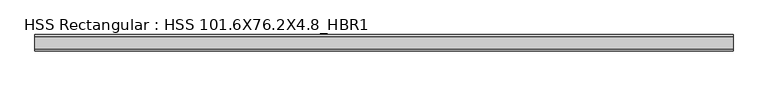
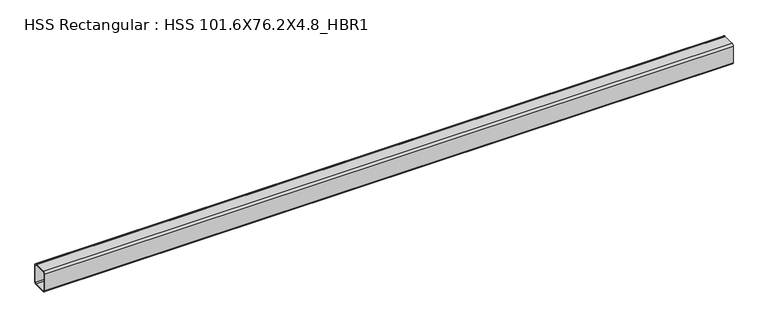
"""IFC4 building model written with IfcOpenShell, lengths in millimetres: beam geometry, HSS Rectangular : HSS 101.6X76.2X4.8_HBR1."""

from ifc_helpers import new_model, si_unit, point, frame, frame_2d, origin, place, context, project, spatial, polyline, circle_curve, trimmed, segment, composite_curve, outline, extrude, source, transform, mapped, element, save


def hss_rectangular_hss_101_6x76_2x4_8_hbr1_9da782e9(model_context):
    return source(origin(), model_context, "Body", "SweptSolid", [
        extrude(outline(composite_curve([segment(polyline([(38.1, 41.275), (38.1, -41.275)]), True, "CONTINUOUS"), segment(trimmed(circle_curve(frame_2d((28.575, -41.275)), 9.525), [point((38.1, -41.275))], [point((28.575, -50.8))], False, "CARTESIAN"), True, "CONTINUOUS"), segment(polyline([(28.575, -50.8), (-28.575, -50.8)]), True, "CONTINUOUS"), segment(trimmed(circle_curve(frame_2d((-28.575, -41.275)), 9.525), [point((-28.575, -50.8))], [point((-38.1, -41.275))], False, "CARTESIAN"), True, "CONTINUOUS"), segment(polyline([(-38.1, -41.275), (-38.1, 41.275)]), True, "CONTINUOUS"), segment(trimmed(circle_curve(frame_2d((-28.575, 41.275)), 9.525), [point((-38.1, 41.275))], [point((-28.575, 50.8))], False, "CARTESIAN"), True, "CONTINUOUS"), segment(polyline([(-28.575, 50.8), (28.575, 50.8)]), True, "CONTINUOUS"), segment(trimmed(circle_curve(frame_2d((28.575, 41.275)), 9.525), [point((28.575, 50.8))], [point((38.1, 41.275))], False, "CARTESIAN"), True, "CONTINUOUS")], self_intersect=False), holes=[composite_curve([segment(trimmed(circle_curve(frame_2d((-28.575, 41.275)), 4.7625), [point((-28.575, 46.0375))], [point((-33.3375, 41.275))], True, "CARTESIAN"), True, "CONTINUOUS"), segment(polyline([(-33.3375, 41.275), (-33.3375, -41.275)]), True, "CONTINUOUS"), segment(trimmed(circle_curve(frame_2d((-28.575, -41.275)), 4.7625), [point((-33.3375, -41.275))], [point((-28.575, -46.0375))], True, "CARTESIAN"), True, "CONTINUOUS"), segment(polyline([(-28.575, -46.0375), (28.575, -46.0375)]), True, "CONTINUOUS"), segment(trimmed(circle_curve(frame_2d((28.575, -41.275)), 4.7625), [point((28.575, -46.0375))], [point((33.3375, -41.275))], True, "CARTESIAN"), True, "CONTINUOUS"), segment(polyline([(33.3375, -41.275), (33.3375, 41.275)]), True, "CONTINUOUS"), segment(trimmed(circle_curve(frame_2d((28.575, 41.275)), 4.7625), [point((33.3375, 41.275))], [point((28.575, 46.0375))], True, "CARTESIAN"), True, "CONTINUOUS"), segment(polyline([(28.575, 46.0375), (-28.575, 46.0375)]), True, "CONTINUOUS")], self_intersect=False)]), frame((-1506.6924156, 0.0, 0.0), z_axis=(1.0, 0.0, 0.0), x_axis=(0.0, 1.0, 0.0)), (0.0, 0.0, 1.0), 3242.2664167),
    ])


if __name__ == "__main__":
    model = new_model("IFC4")
    model_context = context("Model", 3, world=origin())
    ifc_project = project(units=[si_unit("LENGTHUNIT", "METRE", prefix="MILLI")], contexts=[model_context])
    site = spatial("IfcSite", under=ifc_project)
    building = spatial("IfcBuilding", under=site)
    placement = place(None, origin())
    hss_rectangular_hss_101_6x76_2x4_8_hbr1_shape = hss_rectangular_hss_101_6x76_2x4_8_hbr1_9da782e9(model_context)
    element("IfcBeam", 1, ObjectType="HSS Rectangular : HSS 101.6X76.2X4.8_HBR1", at=placement, inside=building, context=model_context, shape_type="MappedRepresentation", body=[
        mapped(hss_rectangular_hss_101_6x76_2x4_8_hbr1_shape, transform((0.0, 0.0, 0.0), x_axis=(1.0, 0.0, 0.0), y_axis=(0.0, 1.0, 0.0), z_axis=(0.0, 0.0, 1.0))),
    ])
    save(model, "model.ifc")

# Revit data of these elements
# Type "HSS Rectangular : HSS 101.6X76.2X4.8_HBR1"
#   Section Name Key = "HSS 4X3X3/16"
#   Assembly Code = "B10"
#   Width = 7.62 cm
#   Wall Nominal Thickness = 0.4763 cm
#   Wall Design Thickness = 0.442 cm
#   Torsional Moment of Inertia = 260.561 cm⁴
#   Torsional Modulus = 61.2876 cm³
#   Section Area = 14.4516 cm²
#   Plastic Modulus weak axis = 40.3122 cm³
#   Plastic Modulus strong axis = 49.1612 cm³
#   Perimeter = 0.881482 m²/m
#   Outer Fillet = 0.9525 cm
#   Nominal Weight = 12.1285 kgf/m
#   Moment of Inertia weak axis = 131.529 cm⁴
#   Moment of Inertia strong axis = 205.202 cm⁴
#   Inner Fillet = 0.4763 cm
#   Height = 10.16 cm
#   Elastic Modulus weak axis = 34.4128 cm³
#   Elastic Modulus strong axis = 40.476 cm³
#   Centroid Vertical = 5.08 cm
#   Centroid Horizontal = 3.81 cm
#   Length [instance default] = 1524 mm
#   Structural Material [instance default] = Steel ASTM A500, Grade B, Rectangular and Square
#   Principal Axes Angle = 0
# Element 1 (IfcBeam, "HSS Rectangular : HSS 101.6X76.2X4.8_HBR1")
#   Structural Material = Steel ASTM A992
#   Materials on its faces: "Steel ASTM A992"
# Materials
#   "Steel ASTM A500, Grade B, Rectangular and Square": class "Metal", colour RGB 199 199 199, transparency 0, Description = "Carbon steel", Cost = 0
#   "Steel ASTM A992": class "Metal", colour RGB 199 199 199, transparency 0, Description = "Structural steel 50ksi", Cost = 0
